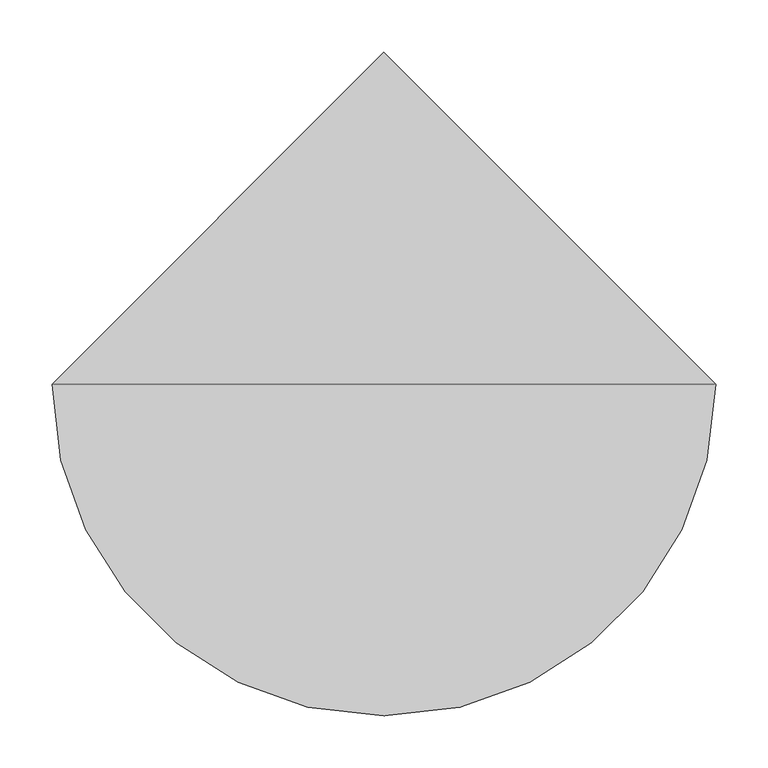
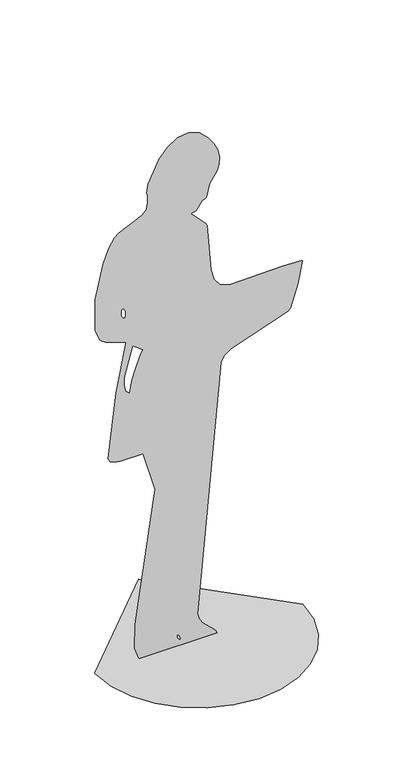
"""IFC4 building model written with IfcOpenShell, lengths in millimetres: proxy geometry, lisa 12 res 26737 : lisa 12 res 26737."""

from ifc_helpers import new_model, si_unit, origin, place, context, project, spatial, triangles, source, transform, mapped, element, save


def entourage_45e033de(model_context):
    return source(origin(), model_context, "Body", "Tessellation", [
        triangles([(-318.6546412, 0.0, 4.24e-05), (-310.2304461, -73.0145749, 4.24e-05), (-286.2384695, -140.0667775, 4.24e-05), (-248.599724, -199.2354951, 4.24e-05), (-199.2355133, -248.5997785, 4.24e-05), (-140.0667412, -286.2383968, 4.24e-05), (-73.0145386, -310.2304461, 4.24e-05), (1.39e-05, -318.6546412, 4.24e-05), (73.014584, -310.2304461, 4.24e-05), (140.0667957, -286.2384331, 4.24e-05), (199.2355133, -248.599724, 4.24e-05), (248.5998148, -199.2355133, 4.24e-05), (286.238415, -140.0667321, 4.24e-05), (310.2304461, -73.0145295, 4.24e-05), (318.6546412, 2.79e-05, 4.24e-05), (-4.18e-05, 318.6546412, 4.24e-05), (-236.0833913, 0.0026468, 1148.558963), (-237.9069355, 0.0026105, 1144.0154903), (-238.9087639, 0.002563, 1138.0610573), (-238.7653679, 0.0025116, 1131.6319439), (-237.1534023, 0.002464, 1125.6650116), (-233.7491951, 0.0024275, 1121.0966858), (-228.2293468, 0.0024096, 1118.8633192), (-225.2501318, 0.002423, 1120.5370543), (-223.8896589, 0.0024609, 1125.2760092), (-225.1557698, 0.0025697, 1138.8987242), (-227.3475873, 0.0026205, 1145.257275), (-230.2886142, 0.0026554, 1149.6301912), (-233.7615672, 0.0026644, 1150.7548319), (-228.8640464, 0.0008634, 925.2704121), (-229.6933199, 0.0006601, 899.8157158), (-224.5596035, 0.0005033, 880.1774523), (-211.6327762, 0.0004187, 869.5889997), (-209.6238145, 0.0005698, 888.5113186), (-204.3871429, 0.0007466, 910.6400551), (-197.1083176, 0.0009324, 933.9116724), (-188.9727495, 0.001111, 956.2624884), (-181.1659404, 0.0012656, 975.6290388), (-174.8732831, 0.00138, 989.9477142), (-171.2802974, 0.0014376, 997.1549778), (-202.5209051, 0.0016247, 1020.5855244), (-66.9848875, -0.00625, 34.6527949), (-67.3190922, -0.0062754, 31.469341), (-66.097746, -0.0063066, 27.5659296), (-61.2032591, -0.0063666, 20.0446749), (-58.6375727, -0.0063858, 17.6494632), (-56.7312301, -0.0063911, 16.9795595), (-55.5294503, -0.0063793, 18.4546012), (-55.6450274, -0.0063551, 21.494868), (-58.5205786, -0.0062906, 29.5655441), (-60.6267682, -0.0062612, 33.2437171), (-62.7426728, -0.0062409, 35.7822068), (-64.5413866, -0.0062352, 36.5050233), (-196.6624146, -0.0062164, 38.8580478), (-195.4353274, -0.0056161, 114.0141163), (-133.7753647, -0.0022844, 531.1485749), (-171.402383, -0.0012522, 660.3822927), (-241.8532245, -0.0012538, 660.1860111), (-258.8309491, -0.0012294, 663.2409845), (-271.6694096, -0.0011781, 669.6640663), (-278.4260648, -0.0010914, 680.5179096), (-253.934809, 0.0005466, 885.5981243), (-223.2260548, 0.0017758, 1039.5006489), (-285.4057623, 0.0019435, 1060.4982771), (-295.9894549, 0.0019962, 1067.1020891), (-303.7276091, 0.0020581, 1074.8495813), (-317.3083571, 0.0023326, 1109.216815), (-317.9938531, 0.0031331, 1209.4468163), (-294.0420992, 0.0039902, 1316.7470982), (-276.8262169, 0.0043352, 1359.9520191), (-258.2498254, 0.0045689, 1389.2086636), (-246.2577703, 0.0046489, 1399.2220058), (-174.1937279, 0.0049131, 1432.3041435), (-163.3074011, 0.0050062, 1443.9612808), (-160.4359739, 0.0050518, 1449.6657291), (-158.1679619, 0.0051123, 1457.2399761), (-156.6086821, 0.005182, 1465.9743267), (-157.2362964, 0.0053902, 1492.0348), (-159.5650241, 0.0054403, 1498.3070915), (-154.8378236, 0.005668, 1526.8146538), (-121.2816596, 0.0062128, 1595.0293854), (-95.2936565, 0.0064508, 1624.823061), (-65.0597234, 0.006613, 1645.1322865), (-32.0003019, 0.0066598, 1650.9999516), (2.4641009, 0.0065518, 1637.4695274), (28.9675133, 0.0063504, 1612.2560955), (47.2368287, 0.0061453, 1586.5784477), (58.1910293, 0.0059436, 1561.3233032), (62.749095, 0.0057523, 1537.3776718), (61.8300514, 0.0055786, 1515.628854), (56.3528375, 0.0054295, 1496.9628422), (33.2519606, 0.00515, 1461.9600368), (23.0950338, 0.0048403, 1423.1935078), (21.6612959, 0.0048225, 1420.962394), (20.9385475, 0.0048135, 1419.837608), (20.4209578, 0.0048099, 1419.3760082), (19.6026757, 0.0048079, 1419.1340172), (17.9778861, 0.0048042, 1418.6690746), (15.0407289, 0.0047952, 1417.5374577), (10.2853756, 0.0047773, 1415.2960247), (-5.5296696, 0.0046024, 1393.3976521), (-9.130582, 0.0045775, 1390.2889755), (-13.8402991, 0.004562, 1388.3415653), (-20.283791, 0.0045566, 1387.6631184), (-23.1512508, 0.0045397, 1385.5520554), (-19.3121706, 0.0044929, 1379.692384), (20.1347857, 0.0041698, 1339.2349697), (25.2754739, 0.0040959, 1329.9816101), (37.7544247, 0.0029161, 1182.2670073), (47.1253212, 0.0026493, 1148.8678104), (64.8741969, 0.0024555, 1124.6021404), (93.9398147, 0.0023655, 1113.3310987), (255.9273654, 0.0024004, 1117.7092472), (313.4802841, 0.002378, 1114.9065113), (317.035009, 0.0023681, 1113.6601484), (317.6680736, 0.0023643, 1113.1853228), (317.9938531, 0.0023603, 1112.6801937), (303.9521956, 0.0018153, 1044.4499107), (280.7535753, 0.001235, 971.7927177), (273.2481287, 0.0011828, 965.2635378), (98.5042527, 0.0007078, 905.7858456), (77.1590167, 0.0005851, 890.419923), (68.2313639, 0.0004395, 872.1924019), (-3.3617688, -0.0058615, 83.2844876), (-0.0366878, -0.0059949, 66.5920109), (8.0270025, -0.0061069, 52.5658866), (19.02897, -0.0062027, 40.5652111), (42.6463658, -0.0063664, 20.0769404), (51.661109, -0.0064444, 10.307415), (56.4127676, -0.0065267, 0.0), (-183.2616518, -0.0065267, 0.0)], [[15, 16, 1], [14, 15, 1], [14, 1, 2], [13, 14, 2], [13, 2, 3], [13, 3, 4], [12, 13, 4], [11, 12, 4], [11, 4, 5], [11, 5, 6], [11, 6, 7], [11, 7, 8], [11, 8, 9], [11, 9, 10], [33, 56, 57], [39, 40, 53], [38, 39, 53], [37, 38, 53], [129, 130, 131], [128, 129, 131], [22, 23, 63], [33, 57, 58], [33, 58, 59], [33, 59, 60], [33, 60, 61], [33, 61, 62], [32, 33, 62], [31, 32, 62], [30, 31, 62], [41, 30, 62], [41, 62, 63], [22, 63, 64], [22, 64, 65], [22, 65, 66], [22, 66, 67], [21, 22, 67], [20, 21, 67], [19, 20, 67], [18, 19, 67], [18, 67, 68], [17, 18, 68], [29, 17, 68], [63, 23, 24], [52, 53, 40], [37, 53, 42], [29, 68, 69], [28, 29, 69], [41, 63, 24], [115, 116, 117], [114, 115, 117], [114, 117, 118], [113, 114, 118], [113, 118, 119], [113, 119, 120], [112, 113, 120], [112, 120, 121], [111, 112, 121], [111, 121, 122], [28, 69, 70], [28, 70, 71], [28, 71, 72], [28, 72, 73], [27, 28, 73], [40, 41, 24], [40, 24, 25], [51, 52, 40], [110, 111, 122], [110, 122, 123], [27, 73, 74], [83, 84, 85], [82, 83, 85], [82, 85, 86], [81, 82, 86], [81, 86, 87], [81, 87, 88], [81, 88, 89], [81, 89, 90], [81, 90, 91], [80, 81, 91], [80, 91, 92], [79, 80, 92], [78, 79, 92], [77, 78, 92], [77, 92, 93], [77, 93, 94], [77, 94, 95], [77, 95, 96], [77, 96, 97], [77, 97, 98], [77, 98, 99], [77, 99, 100], [76, 77, 100], [76, 100, 101], [76, 101, 102], [76, 102, 103], [76, 103, 104], [76, 104, 105], [75, 76, 105], [74, 75, 105], [27, 74, 105], [27, 105, 106], [27, 106, 107], [27, 107, 108], [27, 108, 109], [26, 27, 109], [25, 26, 109], [25, 109, 110], [25, 110, 123], [40, 25, 123], [51, 40, 123], [51, 123, 124], [51, 124, 125], [50, 51, 125], [50, 125, 126], [49, 50, 126], [49, 126, 127], [48, 49, 127], [48, 127, 128], [47, 48, 128], [47, 128, 131], [46, 47, 131], [45, 46, 131], [44, 45, 131], [43, 44, 131], [43, 131, 54], [43, 54, 55], [42, 43, 55], [56, 33, 34], [56, 34, 35], [56, 35, 36], [56, 36, 37], [56, 37, 42], [56, 42, 55]], closed=False),
    ])


if __name__ == "__main__":
    model = new_model("IFC4")
    model_context = context("Model", 3, world=origin())
    ifc_project = project(units=[si_unit("LENGTHUNIT", "METRE", prefix="MILLI")], contexts=[model_context])
    site = spatial("IfcSite", under=ifc_project)
    building = spatial("IfcBuilding", under=site)
    placement = place(None, origin())
    entourage_shape = entourage_45e033de(model_context)
    element("IfcBuildingElementProxy", 1, Name="lisa 12 res 26737 : lisa 12 res 26737", ObjectType="lisa 12 res 26737 : lisa 12 res 26737", at=placement, inside=building, context=model_context, shape_type="MappedRepresentation", body=[
        mapped(entourage_shape, transform((0.0, 0.0, 0.0), x_axis=(1.0, 0.0, 0.0), y_axis=(0.0, 1.0, 0.0), z_axis=(0.0, 0.0, 1.0))),
    ])
    save(model, "model.ifc")

# Revit data of these elements
# Type "lisa 12 res 26737 : lisa 12 res 26737"
#   built-in parameter 1005195 = "RPC-8-N2L1-0HXP-BER1-C"
#   Height = 0
